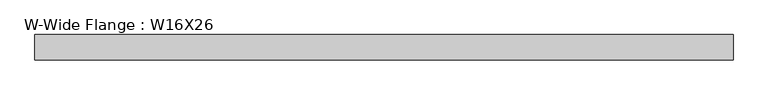
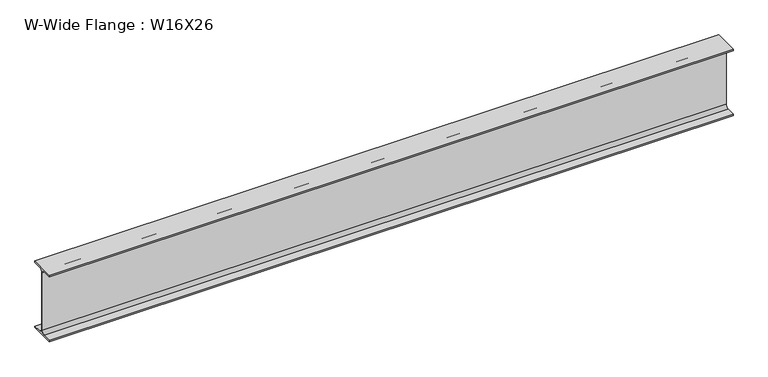
"""IFC4 building model written with IfcOpenShell, lengths in millimetres: beam geometry, W-Wide Flange : W16X26."""

from ifc_helpers import new_model, si_unit, point, frame, frame_2d, origin, place, context, project, spatial, polyline, circle_curve, trimmed, segment, composite_curve, outline, extrude, source, transform, mapped, element, save


def w_wide_flange_w16x26_e3668a51(model_context):
    return source(origin(), model_context, "Body", "SweptSolid", [
        extrude(outline(composite_curve([segment(polyline([(-69.85, -190.5496094), (-21.43125, -190.5496094)]), True, "CONTINUOUS"), segment(trimmed(circle_curve(frame_2d((-21.43125, -172.2933594)), 18.25625), [point((-21.43125, -190.5496094))], [point((-3.175, -172.2933594))], True, "CARTESIAN"), True, "CONTINUOUS"), segment(polyline([(-3.175, -172.2933594), (-3.175, 172.2933594)]), True, "CONTINUOUS"), segment(trimmed(circle_curve(frame_2d((-21.43125, 172.2933594)), 18.25625), [point((-3.175, 172.2933594))], [point((-21.43125, 190.5496094))], True, "CARTESIAN"), True, "CONTINUOUS"), segment(polyline([(-21.43125, 190.5496094), (-69.85, 190.5496094), (-69.85, 199.2808594), (69.85, 199.2808594), (69.85, 190.5496094), (21.43125, 190.5496094)]), True, "CONTINUOUS"), segment(trimmed(circle_curve(frame_2d((21.43125, 172.2933594)), 18.25625), [point((21.43125, 190.5496094))], [point((3.175, 172.2933594))], True, "CARTESIAN"), True, "CONTINUOUS"), segment(polyline([(3.175, 172.2933594), (3.175, -172.2933594)]), True, "CONTINUOUS"), segment(trimmed(circle_curve(frame_2d((21.43125, -172.2933594)), 18.25625), [point((3.175, -172.2933594))], [point((21.43125, -190.5496094))], True, "CARTESIAN"), True, "CONTINUOUS"), segment(polyline([(21.43125, -190.5496094), (69.85, -190.5496094), (69.85, -199.2808594), (-69.85, -199.2808594), (-69.85, -190.5496094)]), True, "CONTINUOUS")], self_intersect=False)), frame((-1892.3, 0.0, 0.0), z_axis=(1.0, 0.0, 0.0), x_axis=(0.0, 1.0, 0.0)), (0.0, 0.0, 1.0), 3873.5),
    ])


if __name__ == "__main__":
    model = new_model("IFC4")
    model_context = context("Model", 3, world=origin())
    ifc_project = project(units=[si_unit("LENGTHUNIT", "METRE", prefix="MILLI")], contexts=[model_context])
    site = spatial("IfcSite", under=ifc_project)
    building = spatial("IfcBuilding", under=site)
    placement = place(None, origin())
    w_wide_flange_w16x26_shape = w_wide_flange_w16x26_e3668a51(model_context)
    element("IfcBeam", 1, ObjectType="W-Wide Flange : W16X26", at=placement, inside=building, context=model_context, shape_type="MappedRepresentation", body=[
        mapped(w_wide_flange_w16x26_shape, transform((0.0, 0.0, 0.0), x_axis=(1.0, 0.0, 0.0), y_axis=(0.0, 1.0, 0.0), z_axis=(0.0, 0.0, 1.0))),
    ])
    save(model, "model.ifc")

# Revit data of these elements
# Type "W-Wide Flange : W16X26"
#   Assembly Code = "B10"
#   W = 26
#   Start Extension Calculation [instance default] = 10' - 0"
#   Start Extension [instance default] = -0' - 0 1/2"
#   End Extension Calculation [instance default] = 10' - 0"
#   End Extension [instance default] = -0' - 0 1/2"
#   Length [instance default] = 5' - 0"
#   bf = 0' - 5 1/2"
#   d = 1' - 3 177/256"
#   k = 0' - 1 1/16"
#   k2 = 0' - 0 23/32"
#   tf = 0' - 0 11/32"
#   tw = 0' - 0 1/4"
#   A = 0.05 SF
#   Beam Material [instance default] = Metal - Steel - ASTM A992
# Element 1 (IfcBeam, "W-Wide Flange : W16X26")
#   Materials on its faces: "Metal - Steel - ASTM A992"
# Materials
#   "Metal - Steel - ASTM A992": class "Metal", colour RGB 128 0 0, transparency 0
